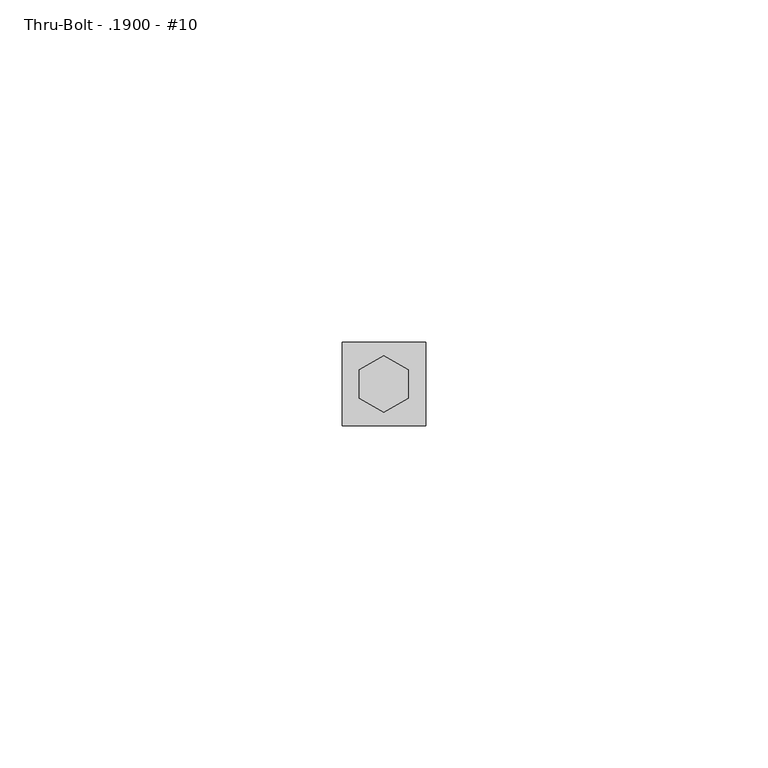
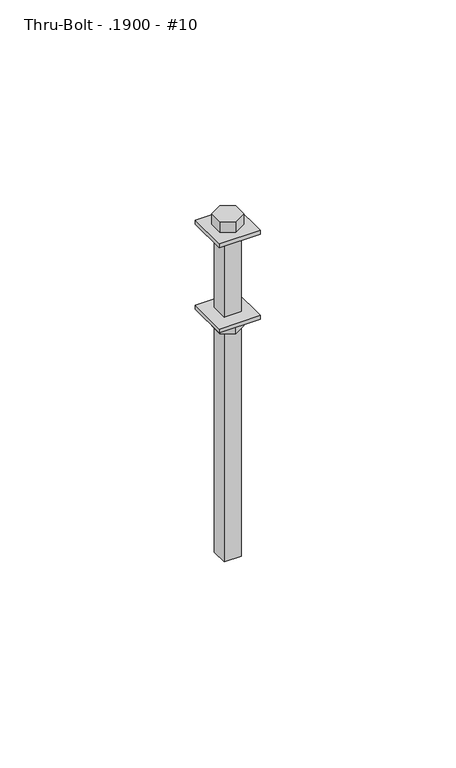
"""IFC4 building model written with IfcOpenShell, lengths in millimetres: fastener geometry, 060523 - W_P_C - Fastenings - Generic - SQUARE : Thru-Bolt - .1900 - #10."""

from ifc_helpers import new_model, si_unit, frame, origin, origin_with_axes, place, context, project, spatial, polyline, outline, extrude, source, transform, mapped, element, save


def thru_bolt_1900_10_c24b497f(model_context):
    return source(origin(), model_context, "Body", "SweptSolid", [
        extrude(outline(polyline([(-6.1019531, -6.1019531), (-6.1019531, 6.1019531), (6.1019531, 6.1019531), (6.1019531, -6.1019531), (-6.1019531, -6.1019531)])), origin_with_axes(), (0.0, 0.0, 1.0), 1.190625),
        extrude(outline(polyline([(-6.1019531, -6.1019531), (-6.1019531, 6.1019531), (6.1019531, 6.1019531), (6.1019531, -6.1019531), (-6.1019531, -6.1019531)])), frame((0.0, 0.0, -26.590625), z_axis=(0.0, 0.0, 1.0), x_axis=(1.0, 0.0, 0.0)), (0.0, 0.0, 1.0), 1.190625),
        extrude(outline(polyline([(-3.571875, -2.062223), (-3.571875, 2.062223), (0.0, 4.124446), (3.571875, 2.062223), (3.571875, -2.062223), (0.0, -4.124446), (-3.571875, -2.062223)])), frame((0.0, 0.0, -30.1625), z_axis=(0.0, 0.0, 1.0), x_axis=(1.0, 0.0, 0.0)), (0.0, 0.0, 1.0), 3.571875),
        extrude(outline(polyline([(-3.571875, 2.062223), (0.0, 4.124446), (3.571875, 2.062223), (3.571875, -2.062223), (0.0, -4.124446), (-3.571875, -2.062223), (-3.571875, 2.062223)])), frame((0.0, 0.0, 1.190625), z_axis=(0.0, 0.0, 1.0), x_axis=(1.0, 0.0, 0.0)), (0.0, 0.0, 1.0), 3.571875),
        extrude(outline(polyline([(-2.5300781, 2.5300781), (2.5300781, 2.5300781), (2.5300781, -2.5300781), (-2.5300781, -2.5300781), (-2.5300781, 2.5300781)])), frame((0.0, 0.0, -101.6), z_axis=(0.0, 0.0, 1.0), x_axis=(1.0, 0.0, 0.0)), (0.0, 0.0, 1.0), 102.790625),
    ])


if __name__ == "__main__":
    model = new_model("IFC4")
    model_context = context("Model", 3, world=origin())
    ifc_project = project(units=[si_unit("LENGTHUNIT", "METRE", prefix="MILLI")], contexts=[model_context])
    site = spatial("IfcSite", under=ifc_project)
    building = spatial("IfcBuilding", under=site)
    placement = place(None, origin())
    thru_bolt_1900_10_shape = thru_bolt_1900_10_c24b497f(model_context)
    element("IfcFastener", 1, ObjectType="060523 - W_P_C - Fastenings - Generic - SQUARE : Thru-Bolt - .1900 - #10", at=placement, inside=building, context=model_context, shape_type="MappedRepresentation", body=[
        mapped(thru_bolt_1900_10_shape, transform((0.0, 0.0, 0.0), x_axis=(1.0, 0.0, 0.0), y_axis=(0.0, 1.0, 0.0), z_axis=(0.0, 0.0, 1.0))),
    ])
    save(model, "model.ifc")

# Revit data of these elements
# Type "060523 - W_P_C - Fastenings - Generic - SQUARE : Thru-Bolt - .1900 - #10"
#   Washer_Thickness = 0' - 0 3/64"
#   Washer Radius = 0' - 0.24023"
#   Washer Offset - Head = 0' - 0 3/64"
#   Washer Offset = 0' - 0 3/64"
#   Thickness_of_Substrate [instance default] = 0' - 1"
#   Side = 0' - 0.1626"
#   Radius = 0' - 0.09961"
#   Length [instance default] = 0' - 4"
#   Head Size = 0' - 0 9/32"
#   Head Radius = 0' - 0 9/64"
#   Head Height = 0' - 0 9/64"
#   Double Diameter = 0' - 0 51/128"
#   Diameter = 0' - 0 51/256"
#   Default Elevation = 4' - 0"
#   Washer_Nut_Visibility = yes
#   Washer_Head_Visibility = yes
#   Round_Head_Visibility = no
#   Point Visibility = no
#   Nut_Visibility = yes
#   Hex_Head_Visiblilty = yes
#   Washer Material = none
#   Bolt Material (Size) = AT SILL - FASTENER AT 24" O.C.
# Element 1 (IfcFastener, "060523 - W_P_C - Fastenings - Generic - SQUARE : Thru-Bolt - .1900 - #10")
#   Materials on its faces: "AT SILL - FASTENER AT 24\" O.C."
# Materials
#   "AT SILL - FASTENER AT 24\" O.C.": class "Generic", colour RGB 120 120 120, transparency 0, Cost = 0
